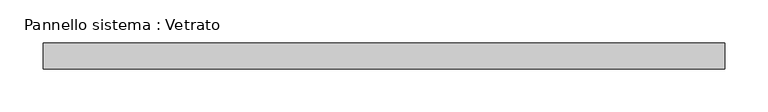
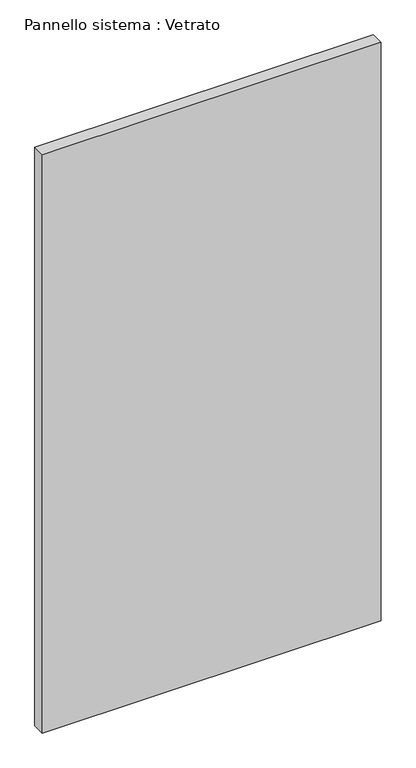
"""IFC4 building model written with IfcOpenShell, lengths in millimetres: plate geometry, Pannello sistema : Vetrato."""

from ifc_helpers import new_model, si_unit, origin, origin_with_axes, place, context, project, spatial, polyline, outline, extrude, source, transform, mapped, element, save


def pannello_sistema_vetrato_b20ec7b4(model_context):
    return source(origin(), model_context, "Body", "SweptSolid", [
        extrude(outline(polyline([(395.0, -15.0), (-395.0, -15.0), (-395.0, 15.0), (395.0, 15.0), (395.0, -15.0)])), origin_with_axes(), (0.0, 0.0, 1.0), 1425.0),
    ])


if __name__ == "__main__":
    model = new_model("IFC4")
    model_context = context("Model", 3, world=origin())
    ifc_project = project(units=[si_unit("LENGTHUNIT", "METRE", prefix="MILLI")], contexts=[model_context])
    site = spatial("IfcSite", under=ifc_project)
    building = spatial("IfcBuilding", under=site)
    placement = place(None, origin())
    pannello_sistema_vetrato_shape = pannello_sistema_vetrato_b20ec7b4(model_context)
    element("IfcPlate", 1, ObjectType="Pannello sistema : Vetrato", at=placement, inside=building, context=model_context, shape_type="MappedRepresentation", body=[
        mapped(pannello_sistema_vetrato_shape, transform((0.0, 0.0, 0.0), x_axis=(1.0, 0.0, 0.0), y_axis=(0.0, 1.0, 0.0), z_axis=(0.0, 0.0, 1.0))),
    ])
    save(model, "model.ifc")

# Revit data of these elements
# Type "Pannello sistema : Vetrato"
#   Construction Type Id = "GSP4R"
#   Analytic Construction = "Vetrata singola Pilkington 1/8 in"
#   Visual Light Transmittance = 0.9
#   Solar Heat Gain Coefficient = 0.86
#   Heat Transfer Coefficient (U) = 6.7069 W/(m²·K)
# Element 1 (IfcPlate, "Pannello sistema : Vetrato")
#   Materials on its faces: "Default - Vetro"
# Materials
#   "Default - Vetro": class "Vetro", colour RGB 208 208 208, transparency 0.7, Cost = 0
